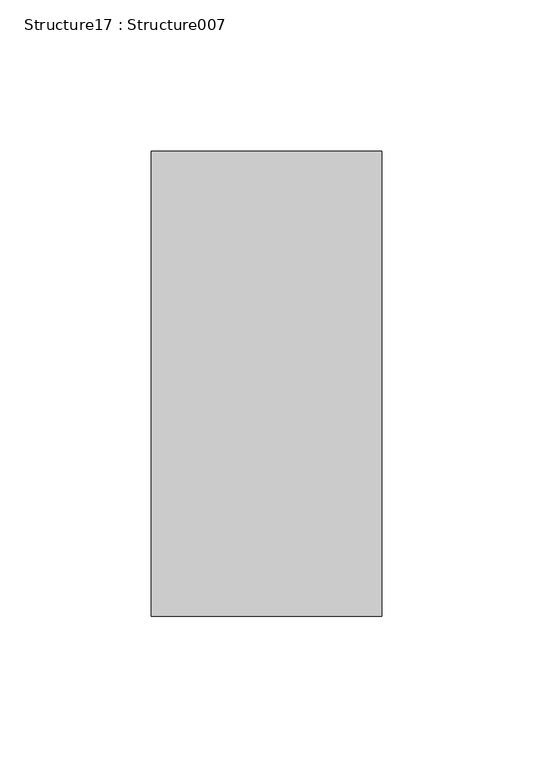
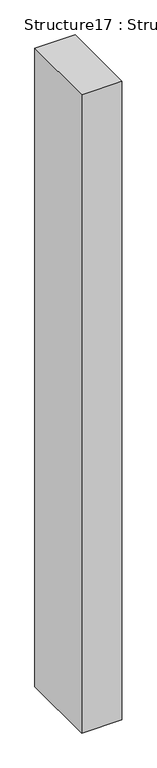
"""IFC4 building model written with IfcOpenShell, lengths in millimetres: proxy geometry, Structure17 : Structure007."""

from ifc_helpers import new_model, si_unit, frame, origin, place, context, project, spatial, polyline, outline, extrude, source, transform, mapped, element, save


def structure17_structure007_4f865c3a(model_context):
    return source(origin(), model_context, "Body", "SweptSolid", [
        extrude(outline(polyline([(0.0, -153.6692087), (0.0, 0.0), (76.2, 0.0), (76.2, -153.6692087), (0.0, -153.6692087)])), frame((-35547.8862846, 277188.9235379, 4479.6663888), z_axis=(-1.3571366253017914e-12, 0.0, 1.0), x_axis=(-1.0, 0.0, -1.3571366253017914e-12)), (0.0, 0.0, 1.0), 1280.4310236),
    ])


if __name__ == "__main__":
    model = new_model("IFC4")
    model_context = context("Model", 3, world=origin())
    ifc_project = project(units=[si_unit("LENGTHUNIT", "METRE", prefix="MILLI")], contexts=[model_context])
    site = spatial("IfcSite", under=ifc_project)
    building = spatial("IfcBuilding", under=site)
    placement = place(None, origin())
    structure17_structure007_shape = structure17_structure007_4f865c3a(model_context)
    element("IfcBuildingElementProxy", 1, Name="Structure17 : Structure007", ObjectType="Structure17 : Structure007", at=placement, inside=building, context=model_context, shape_type="MappedRepresentation", body=[
        mapped(structure17_structure007_shape, transform((0.0, 0.0, 0.0), x_axis=(1.0, 0.0, 0.0), y_axis=(0.0, 1.0, 0.0), z_axis=(0.0, 0.0, 1.0))),
    ])
    save(model, "model.ifc")

# Revit data of these elements
# Type "Structure17 : Structure007"
#   NameOverride = "Structure007"
# Element 1 (IfcBuildingElementProxy, "Structure17 : Structure007")
#   Materials on its faces: "BRUSHED ALUMINUM LETTERING"
# Materials
#   "BRUSHED ALUMINUM LETTERING": class "Unassigned", colour RGB 169 181 186, transparency 0, Cost = 0
